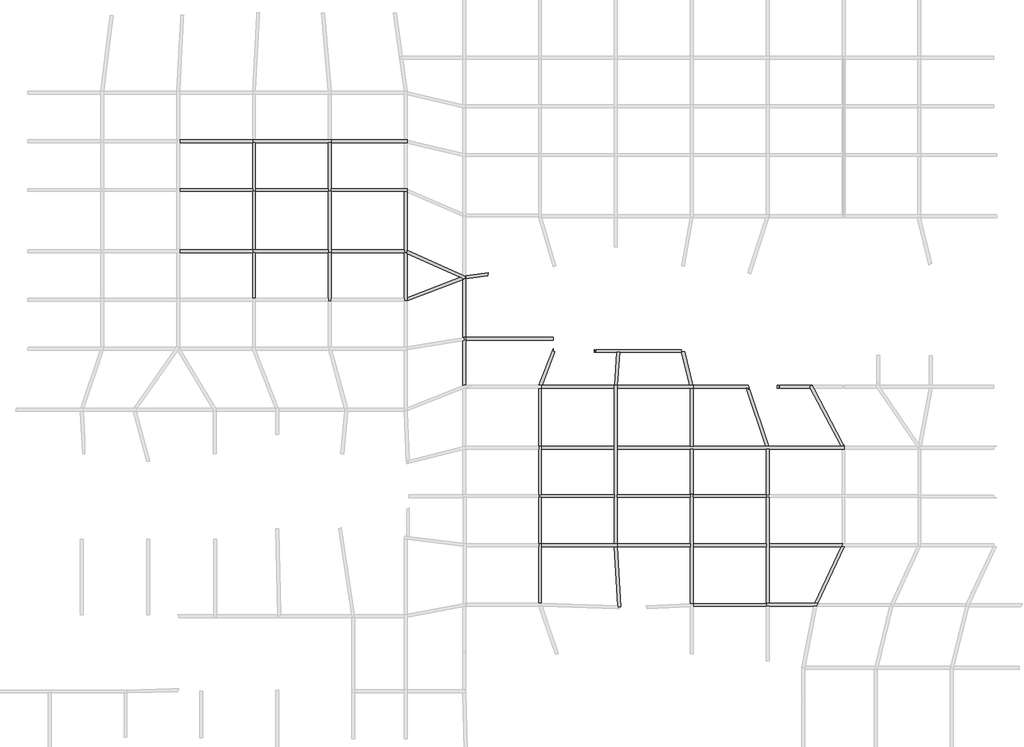
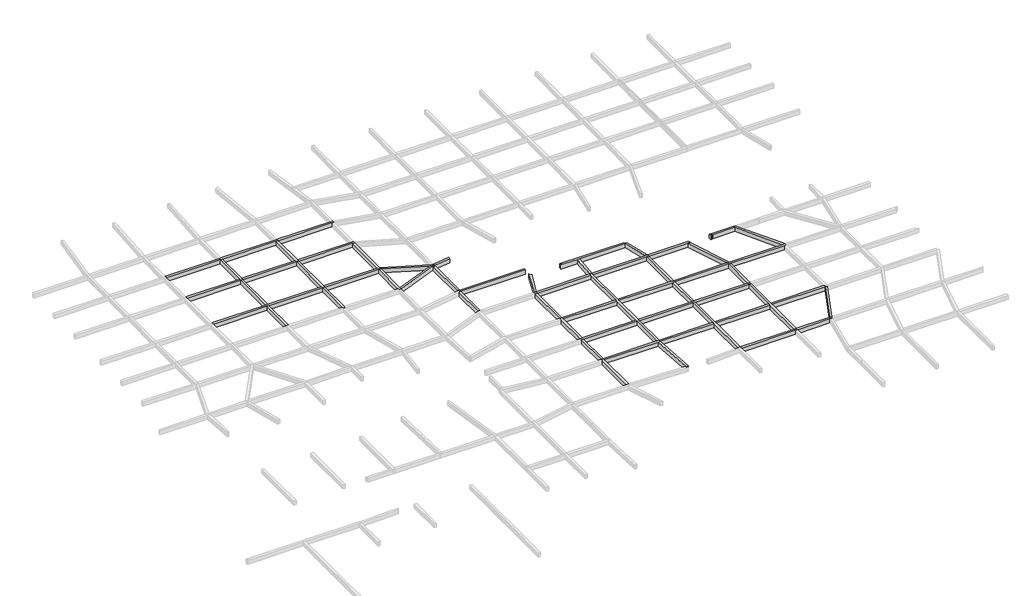
# One storey, part 7 of 15: 54 beams.
"""IFC4 building model written with IfcOpenShell, lengths in millimetres."""

from ifc_helpers import new_model, si_unit, frame, origin, place, context, project, spatial, polyline, outline, extrude, faceted_brep, element, save

model = new_model("IFC4")

# Units and contexts
model_context = context("Model", 3, world=origin())
ifc_project = project(units=[si_unit("LENGTHUNIT", "METRE", prefix="MILLI")], contexts=[model_context])

# Site, building, storey
site = spatial("IfcSite", under=ifc_project)
building = spatial("IfcBuilding", under=site)
storey = spatial("IfcBuildingStorey", under=building, Name="层高", Elevation=3300.0)

# Beams
placement = place(None, origin())
element("IfcBeam", 1, ObjectType="混凝土 - 矩形梁 : KL_beam", at=placement, inside=storey, context=model_context, shape_type="Brep", body=[
    faceted_brep([(161650.300938, 70392.1684205, 3300.0), (161350.300938, 70392.1684205, 3300.0), (161350.300938, 70092.1684205, 3300.0), (161350.300938, 64256.5260367, 3300.0), (161650.300938, 64256.5260367, 3300.0), (161650.300938, 70092.1684205, 3300.0), (161350.300938, 70392.1684205, 2700.0), (161350.300938, 70092.1684205, 2700.0), (161350.300938, 64256.5260367, 2700.0), (161650.300938, 70392.1684205, 2700.0), (161650.300938, 70092.1684205, 2700.0), (161650.300938, 64256.5260367, 2700.0)], [[[0, 1, 2, 3, 4, 5]], [[1, 6, 7, 8, 3, 2]], [[6, 9, 10, 11, 8, 7]], [[9, 0, 5, 4, 11, 10]], [[4, 3, 8, 11]], [[1, 0, 9, 6]]]),
])
element("IfcBeam", 2, ObjectType="混凝土 - 矩形梁 : KL_beam", at=placement, inside=storey, context=model_context, shape_type="Brep", body=[
    faceted_brep([(169458.3679569, 70092.1684205, 3300.0), (169450.3009381, 70246.0963088, 3300.0), (169442.6456231, 70392.1684205, 3300.0), (169150.3009381, 70392.1684205, 3300.0), (161650.300938, 70392.1684205, 3300.0), (161650.300938, 70092.1684205, 3300.0), (169157.9562531, 70092.1684205, 3300.0), (169458.3679569, 70092.1684205, 2700.0), (161650.300938, 70092.1684205, 2700.0), (169157.9562531, 70092.1684205, 2700.0), (169442.6456231, 70392.1684205, 2700.0), (169450.3009381, 70246.0963088, 2700.0), (161650.300938, 70392.1684205, 2700.0), (169150.3009381, 70392.1684205, 2700.0)], [[[0, 1, 2, 3, 4, 5, 6]], [[7, 0, 6, 5, 8, 9]], [[10, 11, 7, 9, 8, 12, 13]], [[2, 10, 13, 12, 4, 3]], [[5, 4, 12, 8]], [[2, 1, 0, 7, 11, 10]]]),
])
element("IfcBeam", 3, ObjectType="混凝土 - 矩形梁 : KL_beam", at=placement, inside=storey, context=model_context, shape_type="Brep", body=[
    faceted_brep([(169458.3679569, 70092.1684205, 3300.0), (169157.9562531, 70092.1684205, 3300.0), (169477.2686164, 63999.3255706, 3300.0), (169481.9445066, 63910.1042703, 3300.0), (169782.3562104, 63910.1042703, 3300.0), (169157.9562531, 70092.1684205, 2700.0), (169477.2686164, 63999.3255706, 2700.0), (169481.9445066, 63910.1042703, 2700.0), (169458.3679569, 70092.1684205, 2700.0), (169782.3562104, 63910.1042703, 2700.0)], [[[0, 1, 2, 3, 4]], [[1, 5, 6, 7, 3, 2]], [[5, 8, 9, 7, 6]], [[8, 0, 4, 9]], [[1, 0, 8, 5]], [[4, 3, 7, 9]]]),
])
element("IfcBeam", 4, ObjectType="混凝土 - 矩形梁 : KL_beam", at=placement, inside=storey, context=model_context, shape_type="Brep", body=[
    faceted_brep([(184765.5848537, 64245.2581831, 3300.0), (184765.5848537, 64242.1684205, 3300.0), (184765.5848537, 63945.2581831, 3300.0), (185065.5848537, 63945.2581831, 3300.0), (189579.4798373, 63945.2581831, 3300.0), (189910.8814312, 63945.2581831, 3300.0), (190050.2396546, 64242.1684205, 3300.0), (190051.6898701, 64245.2581831, 3300.0), (189720.2882761, 64245.2581831, 3300.0), (185065.5848537, 64245.2581831, 3300.0), (184765.5848537, 64245.2581831, 2700.0), (190051.6898701, 64245.2581831, 2700.0), (189720.2882761, 64245.2581831, 2700.0), (185065.5848537, 64245.2581831, 2700.0), (184765.5848537, 63945.2581831, 2700.0), (184765.5848537, 64242.1684205, 2700.0), (190050.2396546, 64242.1684205, 2700.0), (189910.8814312, 63945.2581831, 2700.0), (189579.4798373, 63945.2581831, 2700.0), (185065.5848537, 63945.2581831, 2700.0)], [[[0, 1, 2, 3, 4, 5, 6, 7, 8, 9]], [[10, 0, 9, 8, 7, 11, 12, 13]], [[14, 15, 10, 13, 12, 11, 16, 17, 18, 19]], [[2, 14, 19, 18, 17, 5, 4, 3]], [[2, 1, 0, 10, 15, 14]], [[7, 6, 5, 17, 16, 11]]]),
])
element("IfcBeam", 5, ObjectType="混凝土 - 矩形梁 : KL_beam", at=placement, inside=storey, context=model_context, shape_type="Brep", body=[
    faceted_brep([(184765.5848537, 64245.2581831, 3300.0), (185065.5848537, 64245.2581831, 3300.0), (185065.5848537, 70090.9378389, 3300.0), (185065.5848537, 70390.9378389, 3300.0), (185065.5848537, 75145.2581831, 3300.0), (184765.5848537, 75145.2581831, 3300.0), (184765.5848537, 70392.1684205, 3300.0), (184765.5848537, 70092.1684205, 3300.0), (185065.5848537, 64245.2581831, 2700.0), (185065.5848537, 70090.9378389, 2700.0), (185065.5848537, 70390.9378389, 2700.0), (185065.5848537, 75145.2581831, 2700.0), (184765.5848537, 64245.2581831, 2700.0), (184765.5848537, 70092.1684205, 2700.0), (184765.5848537, 70392.1684205, 2700.0), (184765.5848537, 75145.2581831, 2700.0)], [[[0, 1, 2, 3, 4, 5, 6, 7]], [[1, 8, 9, 10, 11, 4, 3, 2]], [[8, 12, 13, 14, 15, 11, 10, 9]], [[12, 0, 7, 6, 5, 15, 14, 13]], [[1, 0, 12, 8]], [[5, 4, 11, 15]]]),
])
element("IfcBeam", 6, ObjectType="混凝土 - 矩形梁 : KL_beam", at=placement, inside=storey, context=model_context, shape_type="Brep", body=[
    faceted_brep([(185065.5848537, 70390.9378389, 3300.0), (185065.5848537, 70090.9378389, 3300.0), (192464.0250307, 70090.9378389, 3300.0), (192604.8334695, 70390.9378389, 3300.0), (192550.1300471, 70390.9378389, 3300.0), (185065.5848537, 70090.9378389, 2700.0), (192464.0250307, 70090.9378389, 2700.0), (185065.5848537, 70390.9378389, 2700.0), (192550.1300471, 70390.9378389, 2700.0), (192604.8334695, 70390.9378389, 2700.0)], [[[0, 1, 2, 3, 4]], [[1, 5, 6, 2]], [[5, 7, 8, 9, 6]], [[7, 0, 4, 3, 9, 8]], [[1, 0, 7, 5]], [[3, 2, 6, 9]]]),
])
element("IfcBeam", 7, ObjectType="混凝土 - 矩形梁 : KL_beam", at=placement, inside=storey, context=model_context, shape_type="SweptSolid", body=[
    extrude(outline(polyline([(192464.0250307, 70090.9378389), (192795.4266246, 70090.9378389), (190051.6898701, 64245.2581831), (189720.2882761, 64245.2581831), (192464.0250307, 70090.9378389)])), frame((0.0, 0.0, 2700.0), z_axis=(0.0, 0.0, 1.0), x_axis=(1.0, 0.0, 0.0)), (0.0, 0.0, 1.0), 600.0),
])
element("IfcBeam", 8, ObjectType="混凝土 - 矩形梁 : KL_beam", at=placement, inside=storey, context=model_context, shape_type="Brep", body=[
    faceted_brep([(185065.5848537, 63942.1684205, 3300.0), (185065.5848537, 63945.2581831, 3300.0), (184765.5848537, 63945.2581831, 3300.0), (184765.5848537, 64242.1684205, 3300.0), (177250.3009381, 64242.1684205, 3300.0), (177250.3009381, 63942.1684205, 3300.0), (184765.5848537, 63942.1684205, 3300.0), (185065.5848537, 63942.1684205, 2700.0), (177250.3009381, 63942.1684205, 2700.0), (184765.5848537, 63942.1684205, 2700.0), (185065.5848537, 63945.2581831, 2700.0), (177250.3009381, 64242.1684205, 2700.0), (184765.5848537, 64242.1684205, 2700.0), (184765.5848537, 63945.2581831, 2700.0)], [[[0, 1, 2, 3, 4, 5, 6]], [[7, 0, 6, 5, 8, 9]], [[10, 7, 9, 8, 11, 12, 13]], [[3, 12, 11, 4]], [[0, 7, 10, 1]], [[13, 2, 1, 10]], [[2, 13, 12, 3]], [[5, 4, 11, 8]]]),
])
element("IfcBeam", 9, ObjectType="混凝土 - 矩形梁 : KL_beam", at=placement, inside=storey, context=model_context, shape_type="Brep", body=[
    faceted_brep([(176950.3009381, 75492.1684205, 3300.0), (176950.3009381, 75445.2581831, 3300.0), (176950.3009381, 75145.2581831, 3300.0), (176950.3009381, 70392.1684205, 3300.0), (176950.3009381, 70092.1684205, 3300.0), (176950.3009381, 64242.1684205, 3300.0), (177096.3665098, 64242.1684205, 3300.0), (177250.3009381, 64250.249233, 3300.0), (177250.3009381, 70092.1684205, 3300.0), (177250.3009381, 70392.1684205, 3300.0), (177250.3009381, 75145.2581831, 3300.0), (177250.3009381, 75445.2581831, 3300.0), (177250.3009381, 75492.1684205, 3300.0), (177250.3009381, 75492.1684205, 2700.0), (177250.3009381, 64250.249233, 2700.0), (177250.3009381, 70092.1684205, 2700.0), (177250.3009381, 70392.1684205, 2700.0), (177250.3009381, 75145.2581831, 2700.0), (177250.3009381, 75445.2581831, 2700.0), (176950.3009381, 64242.1684205, 2700.0), (176950.3009381, 70092.1684205, 2700.0), (176950.3009381, 70392.1684205, 2700.0), (176950.3009381, 75145.2581831, 2700.0), (176950.3009381, 75445.2581831, 2700.0), (176950.3009381, 75492.1684205, 2700.0), (177096.3665098, 64242.1684205, 2700.0)], [[[0, 1, 2, 3, 4, 5, 6, 7, 8, 9, 10, 11, 12]], [[13, 12, 11, 10, 9, 8, 7, 14, 15, 16, 17, 18]], [[19, 20, 21, 22, 23, 24, 13, 18, 17, 16, 15, 14, 25]], [[5, 4, 3, 2, 1, 0, 24, 23, 22, 21, 20, 19]], [[5, 19, 25, 6]], [[7, 6, 25, 14]], [[0, 12, 13, 24]]]),
])
element("IfcBeam", 10, ObjectType="混凝土 - 矩形梁 : KL_beam", at=placement, inside=storey, context=model_context, shape_type="SweptSolid", body=[
    extrude(outline(polyline([(184765.5848537, 70392.1684205), (184765.5848537, 70092.1684205), (177250.3009381, 70092.1684205), (177250.3009381, 70392.1684205), (184765.5848537, 70392.1684205)])), frame((0.0, 0.0, 2700.0), z_axis=(0.0, 0.0, 1.0), x_axis=(1.0, 0.0, 0.0)), (0.0, 0.0, 1.0), 600.0),
])
element("IfcBeam", 11, ObjectType="混凝土 - 矩形梁 : KL_beam", at=placement, inside=storey, context=model_context, shape_type="Brep", body=[
    faceted_brep([(192790.538789, 80092.1684205, 3300.0), (192790.538789, 80392.1684205, 3300.0), (192451.2603083, 80392.1684205, 3300.0), (185023.3152634, 80392.1684205, 3300.0), (184706.730176, 80392.1684205, 3300.0), (177250.3009381, 80392.1684205, 3300.0), (176950.3009381, 80392.1684205, 3300.0), (169450.3009381, 80392.1684205, 3300.0), (169450.3009381, 80092.1684205, 3300.0), (176950.3009381, 80092.1684205, 3300.0), (177250.3009381, 80092.1684205, 3300.0), (184765.5848537, 80092.1684205, 3300.0), (185065.5848537, 80092.1684205, 3300.0), (192550.1300471, 80092.1684205, 3300.0), (192790.538789, 80392.1684205, 2700.0), (192451.2603083, 80392.1684205, 2700.0), (185023.3152634, 80392.1684205, 2700.0), (184706.730176, 80392.1684205, 2700.0), (177250.3009381, 80392.1684205, 2700.0), (176950.3009381, 80392.1684205, 2700.0), (169450.3009381, 80392.1684205, 2700.0), (192790.538789, 80092.1684205, 2700.0), (192550.1300471, 80092.1684205, 2700.0), (185065.5848537, 80092.1684205, 2700.0), (184765.5848537, 80092.1684205, 2700.0), (177250.3009381, 80092.1684205, 2700.0), (176950.3009381, 80092.1684205, 2700.0), (169450.3009381, 80092.1684205, 2700.0)], [[[0, 1, 2, 3, 4, 5, 6, 7, 8, 9, 10, 11, 12, 13]], [[1, 14, 15, 16, 17, 18, 19, 20, 7, 6, 5, 4, 3, 2]], [[14, 21, 22, 23, 24, 25, 26, 27, 20, 19, 18, 17, 16, 15]], [[21, 0, 13, 12, 11, 10, 9, 8, 27, 26, 25, 24, 23, 22]], [[8, 7, 20, 27]], [[0, 21, 14, 1]]]),
])
element("IfcBeam", 12, ObjectType="混凝土 - 矩形梁 : KL_beam", at=placement, inside=storey, context=model_context, shape_type="SweptSolid", body=[
    extrude(outline(polyline([(177250.3009381, 75492.1684205), (176950.3009381, 75492.1684205), (176950.3009381, 80092.1684205), (177250.3009381, 80092.1684205), (177250.3009381, 75492.1684205)])), frame((0.0, 0.0, 2700.0), z_axis=(0.0, 0.0, 1.0), x_axis=(1.0, 0.0, 0.0)), (0.0, 0.0, 1.0), 600.0),
])
element("IfcBeam", 13, ObjectType="混凝土 - 矩形梁 : KL_beam", at=placement, inside=storey, context=model_context, shape_type="SweptSolid", body=[
    extrude(outline(polyline([(184765.5848537, 80092.1684205), (185065.5848537, 80092.1684205), (185065.5848537, 75445.2581831), (184765.5848537, 75445.2581831), (184765.5848537, 80092.1684205)])), frame((0.0, 0.0, 2700.0), z_axis=(0.0, 0.0, 1.0), x_axis=(1.0, 0.0, 0.0)), (0.0, 0.0, 1.0), 600.0),
])
element("IfcBeam", 14, ObjectType="混凝土 - 矩形梁 : KL_beam", at=placement, inside=storey, context=model_context, shape_type="Brep", body=[
    faceted_brep([(169150.3009381, 70392.1684205, 3300.0), (169442.6456231, 70392.1684205, 3300.0), (169450.3009381, 70246.0963088, 3300.0), (169450.3009381, 70392.1684205, 3300.0), (169450.3009381, 75145.2581831, 3300.0), (169450.3009381, 75445.2581831, 3300.0), (169450.3009381, 80092.1684205, 3300.0), (169450.3009381, 80392.1684205, 3300.0), (169450.3009381, 86368.5594398, 3300.0), (169450.3009381, 86668.5594398, 3300.0), (169160.4236752, 86668.5594398, 3300.0), (169150.3009381, 86668.5594398, 3300.0), (169150.3009381, 86368.5594398, 3300.0), (169150.3009381, 80384.9176514, 3300.0), (169150.3009381, 80084.9176514, 3300.0), (169150.3009381, 75445.2581831, 3300.0), (169150.3009381, 75145.2581831, 3300.0), (169150.3009381, 70392.1684205, 2700.0), (169150.3009381, 86668.5594398, 2700.0), (169150.3009381, 86368.5594398, 2700.0), (169150.3009381, 80384.9176514, 2700.0), (169150.3009381, 80084.9176514, 2700.0), (169150.3009381, 75445.2581831, 2700.0), (169150.3009381, 75145.2581831, 2700.0), (169442.6456231, 70392.1684205, 2700.0), (169160.4236752, 86668.5594398, 2700.0), (169450.3009381, 86668.5594398, 2700.0), (169450.3009381, 86368.5594398, 2700.0), (169450.3009381, 80392.1684205, 2700.0), (169450.3009381, 80092.1684205, 2700.0), (169450.3009381, 75445.2581831, 2700.0), (169450.3009381, 75145.2581831, 2700.0), (169450.3009381, 70392.1684205, 2700.0), (169450.3009381, 70246.0963088, 2700.0)], [[[0, 1, 2, 3, 4, 5, 6, 7, 8, 9, 10, 11, 12, 13, 14, 15, 16]], [[17, 0, 16, 15, 14, 13, 12, 11, 18, 19, 20, 21, 22, 23]], [[24, 17, 23, 22, 21, 20, 19, 18, 25, 26, 27, 28, 29, 30, 31, 32, 33]], [[2, 33, 32, 31, 30, 29, 28, 27, 26, 9, 8, 7, 6, 5, 4, 3]], [[24, 1, 0, 17]], [[1, 24, 33, 2]], [[11, 10, 9, 26, 25, 18]]]),
])
element("IfcBeam", 15, ObjectType="混凝土 - 矩形梁 : KL_beam", at=placement, inside=storey, context=model_context, shape_type="Brep", body=[
    faceted_brep([(184765.5848537, 75145.2581831, 3300.0), (184765.5848537, 75445.2581831, 3300.0), (177250.3009381, 75445.2581831, 3300.0), (177250.3009381, 75145.2581831, 3300.0), (184765.5848537, 75445.2581831, 2700.0), (177250.3009381, 75445.2581831, 2700.0), (184765.5848537, 75145.2581831, 2700.0), (177250.3009381, 75145.2581831, 2700.0)], [[[0, 1, 2, 3]], [[1, 4, 5, 2]], [[4, 6, 7, 5]], [[6, 0, 3, 7]], [[1, 0, 6, 4]], [[3, 2, 5, 7]]]),
    faceted_brep([(176950.3009381, 75445.2581831, 3300.0), (176950.3009381, 75145.2581831, 3300.0), (176950.3009381, 75145.2581831, 2700.0), (176950.3009381, 75445.2581831, 2700.0), (169450.3009381, 75145.2581831, 3300.0), (169450.3009381, 75445.2581831, 3300.0), (169450.3009381, 75445.2581831, 2700.0), (169450.3009381, 75145.2581831, 2700.0)], [[[0, 1, 2, 3]], [[4, 5, 6, 7]], [[1, 0, 5, 4]], [[0, 3, 6, 5]], [[3, 2, 7, 6]], [[2, 1, 4, 7]]]),
    faceted_brep([(161350.300938, 75445.2581831, 3300.0), (161350.300938, 75145.2581831, 3300.0), (161650.300938, 75145.2581831, 3300.0), (169150.3009381, 75145.2581831, 3300.0), (169150.3009381, 75445.2581831, 3300.0), (161650.300938, 75445.2581831, 3300.0), (161350.300938, 75445.2581831, 2700.0), (169150.3009381, 75445.2581831, 2700.0), (161650.300938, 75445.2581831, 2700.0), (161350.300938, 75145.2581831, 2700.0), (169150.3009381, 75145.2581831, 2700.0), (161650.300938, 75145.2581831, 2700.0)], [[[0, 1, 2, 3, 4, 5]], [[6, 0, 5, 4, 7, 8]], [[9, 6, 8, 7, 10, 11]], [[1, 9, 11, 10, 3, 2]], [[4, 3, 10, 7]], [[1, 0, 6, 9]]]),
])
element("IfcBeam", 16, ObjectType="混凝土 - 矩形梁 : KL_beam", at=placement, inside=storey, context=model_context, shape_type="Brep", body=[
    faceted_brep([(161650.300938, 80384.9176514, 3300.0), (161350.300938, 80384.9176514, 3300.0), (161350.300938, 80084.9176514, 3300.0), (161350.300938, 75445.2581831, 3300.0), (161650.300938, 75445.2581831, 3300.0), (161650.300938, 80084.9176514, 3300.0), (161650.300938, 80384.9176514, 2700.0), (161650.300938, 75445.2581831, 2700.0), (161650.300938, 80084.9176514, 2700.0), (161350.300938, 80384.9176514, 2700.0), (161350.300938, 75445.2581831, 2700.0), (161350.300938, 80084.9176514, 2700.0)], [[[0, 1, 2, 3, 4, 5]], [[6, 0, 5, 4, 7, 8]], [[9, 6, 8, 7, 10, 11]], [[1, 9, 11, 10, 3, 2]], [[4, 3, 10, 7]], [[1, 0, 6, 9]]]),
])
element("IfcBeam", 17, ObjectType="混凝土 - 矩形梁 : KL_beam", at=placement, inside=storey, context=model_context, shape_type="SweptSolid", body=[
    extrude(outline(polyline([(161650.300938, 70392.1684205), (161350.300938, 70392.1684205), (161350.300938, 75145.2581831), (161650.300938, 75145.2581831), (161650.300938, 70392.1684205)])), frame((0.0, 0.0, 2700.0), z_axis=(0.0, 0.0, 1.0), x_axis=(1.0, 0.0, 0.0)), (0.0, 0.0, 1.0), 600.0),
])
element("IfcBeam", 18, ObjectType="混凝土 - 矩形梁 : KL_beam", at=placement, inside=storey, context=model_context, shape_type="SweptSolid", body=[
    extrude(outline(polyline([(169458.3679569, 70092.1684205), (169450.3009381, 70246.0963088), (169450.3009381, 70392.1684205), (176950.3009381, 70392.1684205), (176950.3009381, 70092.1684205), (169458.3679569, 70092.1684205)])), frame((0.0, 0.0, 2700.0), z_axis=(0.0, 0.0, 1.0), x_axis=(1.0, 0.0, 0.0)), (0.0, 0.0, 1.0), 600.0),
])
element("IfcBeam", 19, ObjectType="混凝土 - 矩形梁 : KL_beam", at=placement, inside=storey, context=model_context, shape_type="Brep", body=[
    faceted_brep([(131950.3009381, 111892.3894162, 3300.0), (131950.3009381, 111592.3894162, 3300.0), (132250.3009381, 111592.3894162, 3300.0), (139750.3009381, 111592.3894162, 3300.0), (140050.3009381, 111592.3894162, 3300.0), (140050.3009381, 111892.3894162, 3300.0), (139750.3009381, 111892.3894162, 3300.0), (132250.3009381, 111892.3894162, 3300.0), (131950.3009381, 111892.3894162, 2700.0), (140050.3009381, 111892.3894162, 2700.0), (139750.3009381, 111892.3894162, 2700.0), (132250.3009381, 111892.3894162, 2700.0), (131950.3009381, 111592.3894162, 2700.0), (140050.3009381, 111592.3894162, 2700.0), (139750.3009381, 111592.3894162, 2700.0), (132250.3009381, 111592.3894162, 2700.0)], [[[0, 1, 2, 3, 4, 5, 6, 7]], [[8, 0, 7, 6, 5, 9, 10, 11]], [[12, 8, 11, 10, 9, 13, 14, 15]], [[1, 12, 15, 14, 13, 4, 3, 2]], [[1, 0, 8, 12]], [[5, 4, 13, 9]]]),
])
element("IfcBeam", 20, ObjectType="混凝土 - 矩形梁 : KL_beam", at=placement, inside=storey, context=model_context, shape_type="Brep", body=[
    faceted_brep([(131950.3009381, 106592.3894162, 3300.0), (132250.3009381, 106592.3894162, 3300.0), (132250.3009381, 106892.3894162, 3300.0), (132250.3009381, 111592.3894162, 3300.0), (131950.3009381, 111592.3894162, 3300.0), (131950.3009381, 106892.3894162, 3300.0), (132250.3009381, 106592.3894162, 2700.0), (132250.3009381, 106892.3894162, 2700.0), (132250.3009381, 111592.3894162, 2700.0), (131950.3009381, 106592.3894162, 2700.0), (131950.3009381, 106892.3894162, 2700.0), (131950.3009381, 111592.3894162, 2700.0)], [[[0, 1, 2, 3, 4, 5]], [[1, 6, 7, 8, 3, 2]], [[6, 9, 10, 11, 8, 7]], [[9, 0, 5, 4, 11, 10]], [[4, 3, 8, 11]], [[1, 0, 9, 6]]]),
])
element("IfcBeam", 21, ObjectType="混凝土 - 矩形梁 : KL_beam", at=placement, inside=storey, context=model_context, shape_type="Brep", body=[
    faceted_brep([(139750.3009381, 106592.3894162, 3300.0), (140050.3009381, 106592.3894162, 3300.0), (140050.3009381, 106892.3894162, 3300.0), (140050.3009381, 111592.3894162, 3300.0), (139750.3009381, 111592.3894162, 3300.0), (139750.3009381, 106892.3894162, 3300.0), (140050.3009381, 106592.3894162, 2700.0), (140050.3009381, 106892.3894162, 2700.0), (140050.3009381, 111592.3894162, 2700.0), (139750.3009381, 106592.3894162, 2700.0), (139750.3009381, 106892.3894162, 2700.0), (139750.3009381, 111592.3894162, 2700.0)], [[[0, 1, 2, 3, 4, 5]], [[1, 6, 7, 8, 3, 2]], [[6, 9, 10, 11, 8, 7]], [[9, 0, 5, 4, 11, 10]], [[4, 3, 8, 11]], [[1, 0, 9, 6]]]),
])
element("IfcBeam", 22, ObjectType="混凝土 - 矩形梁 : KL_beam", at=placement, inside=storey, context=model_context, shape_type="SweptSolid", body=[
    extrude(outline(polyline([(132250.3009381, 106592.3894162), (132250.3009381, 106892.3894162), (139750.3009381, 106892.3894162), (139750.3009381, 106592.3894162), (132250.3009381, 106592.3894162)])), frame((0.0, 0.0, 2700.0), z_axis=(0.0, 0.0, 1.0), x_axis=(1.0, 0.0, 0.0)), (0.0, 0.0, 1.0), 600.0),
])
element("IfcBeam", 23, ObjectType="混凝土 - 矩形梁 : KL_beam", at=placement, inside=storey, context=model_context, shape_type="Brep", body=[
    faceted_brep([(147850.2032763, 111592.3894162, 3300.0), (147850.2032763, 111861.4143495, 3300.0), (147850.2032763, 111892.3894162, 3300.0), (147550.2032763, 111892.3894162, 3300.0), (140050.3009381, 111892.3894162, 3300.0), (140050.3009381, 111592.3894162, 3300.0), (147550.2032763, 111592.3894162, 3300.0), (147850.2032763, 111892.3894162, 2700.0), (147550.2032763, 111892.3894162, 2700.0), (140050.3009381, 111892.3894162, 2700.0), (147850.2032763, 111861.4143495, 2700.0), (147850.2032763, 111592.3894162, 2700.0), (147550.2032763, 111592.3894162, 2700.0), (140050.3009381, 111592.3894162, 2700.0)], [[[0, 1, 2, 3, 4, 5, 6]], [[2, 7, 8, 9, 4, 3]], [[7, 10, 11, 12, 13, 9, 8]], [[11, 0, 6, 5, 13, 12]], [[5, 4, 9, 13]], [[2, 1, 0, 11, 10, 7]]]),
])
element("IfcBeam", 24, ObjectType="混凝土 - 矩形梁 : KL_beam", at=placement, inside=storey, context=model_context, shape_type="Brep", body=[
    faceted_brep([(147850.2032763, 106592.3894162, 3300.0), (147850.2032763, 106840.5198943, 3300.0), (147850.2032763, 106892.3894162, 3300.0), (147550.2032763, 106892.3894162, 3300.0), (140050.3009381, 106892.3894162, 3300.0), (140050.3009381, 106592.3894162, 3300.0), (147550.2032763, 106592.3894162, 3300.0), (147668.8470787, 106592.3894162, 3300.0), (147850.2032763, 106592.3894162, 2700.0), (140050.3009381, 106592.3894162, 2700.0), (147550.2032763, 106592.3894162, 2700.0), (147668.8470787, 106592.3894162, 2700.0), (147850.2032763, 106892.3894162, 2700.0), (147850.2032763, 106840.5198943, 2700.0), (140050.3009381, 106892.3894162, 2700.0), (147550.2032763, 106892.3894162, 2700.0)], [[[0, 1, 2, 3, 4, 5, 6, 7]], [[8, 0, 7, 6, 5, 9, 10, 11]], [[12, 13, 8, 11, 10, 9, 14, 15]], [[2, 12, 15, 14, 4, 3]], [[5, 4, 14, 9]], [[2, 1, 0, 8, 13, 12]]]),
])
element("IfcBeam", 25, ObjectType="混凝土 - 矩形梁 : KL_beam", at=placement, inside=storey, context=model_context, shape_type="Brep", body=[
    faceted_brep([(147550.2032763, 100292.3894162, 3300.0), (147668.0058777, 100292.3894162, 3300.0), (147850.2032763, 100292.3894162, 3300.0), (147850.2032763, 100539.3742818, 3300.0), (147850.2032763, 106513.1028536, 3300.0), (147668.8470787, 106592.3894162, 3300.0), (147550.2032763, 106592.3894162, 3300.0), (147550.2032763, 100592.3894162, 3300.0), (147550.2032763, 106592.3894162, 2700.0), (147550.2032763, 100592.3894162, 2700.0), (147550.2032763, 100292.3894162, 2700.0), (147850.2032763, 100292.3894162, 2700.0), (147668.0058777, 100292.3894162, 2700.0), (147668.8470787, 106592.3894162, 2700.0), (147850.2032763, 106513.1028536, 2700.0), (147850.2032763, 100539.3742818, 2700.0)], [[[0, 1, 2, 3, 4, 5, 6, 7]], [[6, 8, 9, 10, 0, 7]], [[11, 12, 10, 9, 8, 13, 14, 15]], [[2, 11, 15, 14, 4, 3]], [[8, 6, 5, 13]], [[5, 4, 14, 13]], [[2, 1, 0, 10, 12, 11]]]),
])
element("IfcBeam", 26, ObjectType="混凝土 - 矩形梁 : KL_beam", at=placement, inside=storey, context=model_context, shape_type="Brep", body=[
    faceted_brep([(139750.3009381, 100292.3894162, 3300.0), (140050.3009381, 100292.3894162, 3300.0), (140050.3009381, 100592.3894162, 3300.0), (140050.3009381, 106592.3894162, 3300.0), (139750.3009381, 106592.3894162, 3300.0), (139750.3009381, 100592.3894162, 3300.0), (140050.3009381, 100292.3894162, 2700.0), (140050.3009381, 100592.3894162, 2700.0), (140050.3009381, 106592.3894162, 2700.0), (139750.3009381, 100292.3894162, 2700.0), (139750.3009381, 100592.3894162, 2700.0), (139750.3009381, 106592.3894162, 2700.0)], [[[0, 1, 2, 3, 4, 5]], [[1, 6, 7, 8, 3, 2]], [[6, 9, 10, 11, 8, 7]], [[9, 0, 5, 4, 11, 10]], [[4, 3, 8, 11]], [[1, 0, 9, 6]]]),
])
element("IfcBeam", 27, ObjectType="混凝土 - 矩形梁 : KL_beam", at=placement, inside=storey, context=model_context, shape_type="SweptSolid", body=[
    extrude(outline(polyline([(147550.2032763, 100592.3894162), (147550.2032763, 100292.3894162), (140050.3009381, 100292.3894162), (140050.3009381, 100592.3894162), (147550.2032763, 100592.3894162)])), frame((0.0, 0.0, 2700.0), z_axis=(0.0, 0.0, 1.0), x_axis=(1.0, 0.0, 0.0)), (0.0, 0.0, 1.0), 600.0),
])
element("IfcBeam", 28, ObjectType="混凝土 - 矩形梁 : KL_beam", at=placement, inside=storey, context=model_context, shape_type="Brep", body=[
    faceted_brep([(147850.2032763, 100539.3742818, 3300.0), (147850.2032763, 100292.3894162, 3300.0), (147668.0058777, 100292.3894162, 3300.0), (147850.2032763, 100210.3944563, 3300.0), (153310.1557551, 97753.2321258, 3300.0), (153695.684915, 97579.7310317, 3300.0), (153727.18388, 97565.5554376, 3300.0), (153741.0642282, 97596.3983497, 3300.0), (153741.4601305, 97597.2780667, 3300.0), (153850.3009381, 97839.1284443, 3300.0), (153550.3009381, 97974.1385386, 3300.0), (147668.0058777, 100292.3894162, 2700.0), (147850.2032763, 100210.3944563, 2700.0), (153310.1557551, 97753.2321258, 2700.0), (153695.684915, 97579.7310317, 2700.0), (153727.18388, 97565.5554376, 2700.0), (147850.2032763, 100292.3894162, 2700.0), (147850.2032763, 100539.3742818, 2700.0), (153550.3009381, 97974.1385386, 2700.0), (153850.3009381, 97839.1284443, 2700.0), (153741.4601305, 97597.2780667, 2700.0), (153741.0642282, 97596.3983497, 2700.0)], [[[0, 1, 2, 3, 4, 5, 6, 7, 8, 9, 10]], [[2, 11, 12, 13, 14, 15, 6, 5, 4, 3]], [[16, 17, 18, 19, 20, 21, 15, 14, 13, 12, 11]], [[17, 0, 10, 9, 19, 18]], [[16, 1, 0, 17]], [[1, 16, 11, 2]], [[9, 8, 7, 6, 15, 21, 20, 19]]]),
])
element("IfcBeam", 29, ObjectType="混凝土 - 矩形梁 : KL_beam", at=placement, inside=storey, context=model_context, shape_type="Brep", body=[
    faceted_brep([(147550.2032763, 95338.9797898, 3300.0), (147850.2032763, 95338.9797898, 3300.0), (147850.2032763, 95660.2659592, 3300.0), (147850.2032763, 100210.3944563, 3300.0), (147668.0058777, 100292.3894162, 3300.0), (147550.2032763, 100292.3894162, 3300.0), (147550.2032763, 95592.1233035, 3300.0), (147550.2032763, 100292.3894162, 2700.0), (147550.2032763, 95592.1233035, 2700.0), (147550.2032763, 95338.9797898, 2700.0), (147850.2032763, 95338.9797898, 2700.0), (147668.0058777, 100292.3894162, 2700.0), (147850.2032763, 100210.3944563, 2700.0), (147850.2032763, 95660.2659592, 2700.0)], [[[0, 1, 2, 3, 4, 5, 6]], [[5, 7, 8, 9, 0, 6]], [[10, 9, 8, 7, 11, 12, 13]], [[1, 10, 13, 12, 3, 2]], [[7, 5, 4, 11]], [[4, 3, 12, 11]], [[1, 0, 9, 10]]]),
])
element("IfcBeam", 30, ObjectType="混凝土 - 矩形梁 : KL_beam", at=placement, inside=storey, context=model_context, shape_type="Brep", body=[
    faceted_brep([(139750.3009381, 95292.1233035, 3300.0), (140050.3009381, 95292.1233035, 3300.0), (140050.3009381, 95592.1233035, 3300.0), (140050.3009381, 100292.3894162, 3300.0), (139750.3009381, 100292.3894162, 3300.0), (139750.3009381, 95592.1233035, 3300.0), (139750.3009381, 95292.1233035, 2700.0), (139750.3009381, 100292.3894162, 2700.0), (139750.3009381, 95592.1233035, 2700.0), (140050.3009381, 95292.1233035, 2700.0), (140050.3009381, 100292.3894162, 2700.0), (140050.3009381, 95592.1233035, 2700.0)], [[[0, 1, 2, 3, 4, 5]], [[6, 0, 5, 4, 7, 8]], [[9, 6, 8, 7, 10, 11]], [[1, 9, 11, 10, 3, 2]], [[4, 3, 10, 7]], [[1, 0, 6, 9]]]),
])
element("IfcBeam", 31, ObjectType="混凝土 - 矩形梁 : KL_beam", at=placement, inside=storey, context=model_context, shape_type="Brep", body=[
    faceted_brep([(131950.3009381, 100592.3894162, 3300.0), (131950.3009381, 100292.3894162, 3300.0), (132250.3009381, 100292.3894162, 3300.0), (139750.3009381, 100292.3894162, 3300.0), (139750.3009381, 100592.3894162, 3300.0), (132250.3009381, 100592.3894162, 3300.0), (131950.3009381, 100292.3894162, 2700.0), (132250.3009381, 100292.3894162, 2700.0), (139750.3009381, 100292.3894162, 2700.0), (131950.3009381, 100592.3894162, 2700.0), (132250.3009381, 100592.3894162, 2700.0), (139750.3009381, 100592.3894162, 2700.0)], [[[0, 1, 2, 3, 4, 5]], [[1, 6, 7, 8, 3, 2]], [[6, 9, 10, 11, 8, 7]], [[9, 0, 5, 4, 11, 10]], [[4, 3, 8, 11]], [[1, 0, 9, 6]]]),
])
element("IfcBeam", 32, ObjectType="混凝土 - 矩形梁 : KL_beam", at=placement, inside=storey, context=model_context, shape_type="SweptSolid", body=[
    extrude(outline(polyline([(131950.3009381, 100292.3894162), (132250.3009381, 100292.3894162), (132250.3009381, 95592.1233035), (131950.3009381, 95592.1233035), (131950.3009381, 100292.3894162)])), frame((0.0, 0.0, 2700.0), z_axis=(0.0, 0.0, 1.0), x_axis=(1.0, 0.0, 0.0)), (0.0, 0.0, 1.0), 600.0),
])
element("IfcBeam", 33, ObjectType="混凝土 - 矩形梁 : KL_beam", at=placement, inside=storey, context=model_context, shape_type="SweptSolid", body=[
    extrude(outline(polyline([(131950.3009381, 106592.3894162), (132250.3009381, 106592.3894162), (132250.3009381, 100592.3894162), (131950.3009381, 100592.3894162), (131950.3009381, 106592.3894162)])), frame((0.0, 0.0, 2700.0), z_axis=(0.0, 0.0, 1.0), x_axis=(1.0, 0.0, 0.0)), (0.0, 0.0, 1.0), 600.0),
])
element("IfcBeam", 34, ObjectType="混凝土 - 矩形梁 : KL_beam", at=placement, inside=storey, context=model_context, shape_type="SweptSolid", body=[
    extrude(outline(polyline([(124450.3009381, 100292.3894162), (124450.3009381, 100592.3894162), (131950.3009381, 100592.3894162), (131950.3009381, 100292.3894162), (124450.3009381, 100292.3894162)])), frame((0.0, 0.0, 2700.0), z_axis=(0.0, 0.0, 1.0), x_axis=(1.0, 0.0, 0.0)), (0.0, 0.0, 1.0), 600.0),
])
element("IfcBeam", 35, ObjectType="混凝土 - 矩形梁 : KL_beam", at=placement, inside=storey, context=model_context, shape_type="SweptSolid", body=[
    extrude(outline(polyline([(124450.3009381, 106592.3894162), (124450.3009381, 106892.3894162), (131950.3009381, 106892.3894162), (131950.3009381, 106592.3894162), (124450.3009381, 106592.3894162)])), frame((0.0, 0.0, 2700.0), z_axis=(0.0, 0.0, 1.0), x_axis=(1.0, 0.0, 0.0)), (0.0, 0.0, 1.0), 600.0),
])
element("IfcBeam", 36, ObjectType="混凝土 - 矩形梁 : KL_beam", at=placement, inside=storey, context=model_context, shape_type="Brep", body=[
    faceted_brep([(189203.3917758, 86541.0667552, 3300.0), (189287.8431053, 86381.1826239, 3300.0), (192451.2603083, 80392.1684205, 3300.0), (192790.538789, 80392.1684205, 3300.0), (192711.3752265, 80542.0416967, 3300.0), (192640.3009401, 80542.0416967, 3300.0), (192640.3009401, 80676.6002718, 3300.0), (189627.121586, 86381.1826239, 3300.0), (189468.6605892, 86681.1826239, 3300.0), (189203.3917758, 86541.0667552, 2700.0), (189287.8431053, 86381.1826239, 2700.0), (192451.2603083, 80392.1684205, 2700.0), (189468.6605892, 86681.1826239, 2700.0), (189627.121586, 86381.1826239, 2700.0), (192640.3009401, 80676.6002718, 2700.0), (192640.3009401, 80542.0416967, 2700.0), (192711.3752265, 80542.0416967, 2700.0), (192790.538789, 80392.1684205, 2700.0)], [[[0, 1, 2, 3, 4, 5, 6, 7, 8]], [[2, 1, 0, 9, 10, 11]], [[11, 10, 9, 12, 13, 14, 15, 16, 17]], [[3, 17, 16, 4]], [[3, 2, 11, 17]], [[8, 12, 9, 0]], [[5, 15, 14, 6]], [[15, 5, 4, 16]], [[12, 8, 7, 6, 14, 13]]]),
])
element("IfcBeam", 37, ObjectType="混凝土 - 矩形梁 : KL_beam", at=placement, inside=storey, context=model_context, shape_type="Brep", body=[
    faceted_brep([(153850.3009381, 97639.000065, 2700.0), (153850.3009381, 97639.000065, 3300.0), (153741.4601305, 97597.2780667, 3300.0), (153741.4601305, 97597.2780667, 2700.0), (153850.3009381, 97839.1284443, 2700.0), (153850.3009381, 97839.1284443, 3300.0)], [[[0, 1, 2, 3]], [[1, 0, 4, 5]], [[1, 5, 2]], [[4, 0, 3]], [[2, 5, 4, 3]]]),
    faceted_brep([(153695.684915, 97579.7310317, 3300.0), (153695.684915, 97579.7310317, 2700.0), (153550.3009381, 97645.1587131, 2700.0), (153310.1557551, 97753.2321258, 2700.0), (153310.1557551, 97753.2321258, 3300.0), (153550.3009381, 97645.1587131, 3300.0), (147850.2032763, 95660.2659592, 2700.0), (147850.2032763, 95660.2659592, 3300.0), (147850.2032763, 95338.9797898, 2700.0), (147850.2032763, 95338.9797898, 3300.0), (153550.3009381, 97524.0009231, 3300.0), (153550.3009381, 97524.0009231, 2700.0)], [[[0, 1, 2, 3, 4, 5]], [[4, 3, 6, 7]], [[7, 6, 8, 9]], [[9, 10, 0, 5, 4, 7]], [[0, 10, 9, 8, 11, 1]], [[1, 11, 8, 6, 3, 2]]]),
])
element("IfcBeam", 38, ObjectType="混凝土 - 矩形梁 : KL_beam", at=placement, inside=storey, context=model_context, shape_type="Brep", body=[
    faceted_brep([(156166.4670288, 98240.2147555, 2700.0), (156166.4670288, 98240.2147555, 3300.0), (156179.085005, 98150.4331897, 3300.0), (156179.085005, 98150.4331897, 2700.0), (153850.3009381, 97914.6988398, 3300.0), (153850.3009381, 97839.1284443, 3300.0), (153850.3009381, 97639.000065, 3300.0), (153741.4601305, 97597.2780667, 3300.0), (153741.0642282, 97596.3983497, 3300.0), (153850.3009381, 97611.750568, 3300.0), (156127.8219291, 97931.8352692, 3300.0), (156127.8219291, 98150.4331897, 3300.0), (153741.0642282, 97596.3983497, 2700.0), (153850.3009381, 97611.750568, 2700.0), (156127.8219291, 97931.8352692, 2700.0), (153850.3009381, 97914.6988398, 2700.0), (156127.8219291, 98150.4331897, 2700.0), (153741.4601305, 97597.2780667, 2700.0), (153850.3009381, 97639.000065, 2700.0), (153850.3009381, 97839.1284443, 2700.0)], [[[0, 1, 2, 3]], [[1, 4, 5, 6, 7, 8, 9, 10, 11, 2]], [[8, 12, 13, 14, 10, 9]], [[15, 0, 3, 16, 14, 13, 12, 17, 18, 19]], [[1, 0, 15, 4]], [[12, 8, 7, 17]], [[4, 15, 19, 18, 6, 5]], [[6, 18, 17, 7]], [[16, 11, 10, 14]], [[11, 16, 3, 2]]]),
])
element("IfcBeam", 39, ObjectType="混凝土 - 矩形梁 : KL_beam", at=placement, inside=storey, context=model_context, shape_type="SweptSolid", body=[
    extrude(outline(polyline([(153695.684915, 97579.7310317), (153727.18388, 97565.5554376), (153741.0642282, 97596.3983497), (153850.3009381, 97611.750568), (153850.3009381, 91592.168885), (153687.8894584, 91592.168885), (153550.3009381, 91569.2428953), (153550.3009381, 97524.0009231), (153695.684915, 97579.7310317)])), frame((0.0, 0.0, 2700.0), z_axis=(0.0, 0.0, 1.0), x_axis=(1.0, 0.0, 0.0)), (0.0, 0.0, 1.0), 600.0),
])
element("IfcBeam", 40, ObjectType="混凝土 - 矩形梁 : KL_beam", at=placement, inside=storey, context=model_context, shape_type="SweptSolid", body=[
    extrude(outline(polyline([(124450.3009381, 111592.3894162), (124450.3009381, 111892.3894162), (131950.3009381, 111892.3894162), (131950.3009381, 111592.3894162), (124450.3009381, 111592.3894162)])), frame((0.0, 0.0, 2700.0), z_axis=(0.0, 0.0, 1.0), x_axis=(1.0, 0.0, 0.0)), (0.0, 0.0, 1.0), 600.0),
])
element("IfcBeam", 41, ObjectType="混凝土 - 矩形梁 : KL_beam", at=placement, inside=storey, context=model_context, shape_type="SweptSolid", body=[
    extrude(outline(polyline([(161350.300938, 86368.5594398), (161650.300938, 86368.5594398), (161650.300938, 80384.9176514), (161350.300938, 80384.9176514), (161350.300938, 86368.5594398)])), frame((0.0, 0.0, 2700.0), z_axis=(0.0, 0.0, 1.0), x_axis=(1.0, 0.0, 0.0)), (0.0, 0.0, 1.0), 600.0),
])
element("IfcBeam", 42, ObjectType="混凝土 - 矩形梁 : KL_beam", at=placement, inside=storey, context=model_context, shape_type="SweptSolid", body=[
    extrude(outline(polyline([(161650.300938, 80084.9176514), (161650.300938, 80384.9176514), (169150.3009381, 80384.9176514), (169150.3009381, 80084.9176514), (161650.300938, 80084.9176514)])), frame((0.0, 0.0, 2700.0), z_axis=(0.0, 0.0, 1.0), x_axis=(1.0, 0.0, 0.0)), (0.0, 0.0, 1.0), 600.0),
])
element("IfcBeam", 43, ObjectType="混凝土 - 矩形梁 : KL_beam", at=placement, inside=storey, context=model_context, shape_type="Brep", body=[
    faceted_brep([(169150.3009381, 86368.5594398, 3300.0), (169150.3009381, 86668.5594398, 3300.0), (161718.5522923, 86668.5594398, 3300.0), (161650.300938, 86668.5594398, 3300.0), (161650.300938, 86368.5594398, 3300.0), (169150.3009381, 86368.5594398, 2700.0), (161650.300938, 86368.5594398, 2700.0), (169150.3009381, 86668.5594398, 2700.0), (161650.300938, 86668.5594398, 2700.0), (161718.5522923, 86668.5594398, 2700.0)], [[[0, 1, 2, 3, 4]], [[5, 0, 4, 6]], [[7, 5, 6, 8, 9]], [[1, 7, 9, 8, 3, 2]], [[1, 0, 5, 7]], [[4, 3, 8, 6]]]),
])
element("IfcBeam", 44, ObjectType="混凝土 - 矩形梁 : KL_beam", at=placement, inside=storey, context=model_context, shape_type="Brep", body=[
    faceted_brep([(177250.3009381, 86368.5594398, 3300.0), (177250.3009381, 86668.5594398, 3300.0), (177217.4937821, 86668.5594398, 3300.0), (176908.3096933, 86668.5594398, 3300.0), (169461.1562446, 86668.5594398, 3300.0), (169450.3009381, 86668.5594398, 3300.0), (169450.3009381, 86368.5594398, 3300.0), (176950.3009381, 86368.5594398, 3300.0), (177250.3009381, 86368.5594398, 2700.0), (169450.3009381, 86368.5594398, 2700.0), (176950.3009381, 86368.5594398, 2700.0), (177250.3009381, 86668.5594398, 2700.0), (169450.3009381, 86668.5594398, 2700.0), (169461.1562446, 86668.5594398, 2700.0), (176908.3096933, 86668.5594398, 2700.0), (177217.4937821, 86668.5594398, 2700.0)], [[[0, 1, 2, 3, 4, 5, 6, 7]], [[8, 0, 7, 6, 9, 10]], [[11, 8, 10, 9, 12, 13, 14, 15]], [[1, 11, 15, 14, 13, 12, 5, 4, 3, 2]], [[6, 5, 12, 9]], [[1, 0, 8, 11]]]),
])
element("IfcBeam", 45, ObjectType="混凝土 - 矩形梁 : KL_beam", at=placement, inside=storey, context=model_context, shape_type="Brep", body=[
    faceted_brep([(183008.7880416, 86368.5594398, 3300.0), (182907.6637736, 86668.5594398, 3300.0), (177250.3009381, 86668.5594398, 3300.0), (177250.3009381, 86368.5594398, 3300.0), (182692.2029542, 86368.5594398, 3300.0), (182840.4077224, 86368.5594398, 3300.0), (182960.4077224, 86368.5594398, 3300.0), (183008.7880416, 86368.5594398, 2700.0), (177250.3009381, 86368.5594398, 2700.0), (182692.2029542, 86368.5594398, 2700.0), (182840.4077224, 86368.5594398, 2700.0), (182960.4077224, 86368.5594398, 2700.0), (182907.6637736, 86668.5594398, 2700.0), (177250.3009381, 86668.5594398, 2700.0)], [[[0, 1, 2, 3, 4, 5, 6]], [[7, 0, 6, 5, 4, 3, 8, 9, 10, 11]], [[12, 7, 11, 10, 9, 8, 13]], [[1, 12, 13, 2]], [[3, 2, 13, 8]], [[1, 0, 7, 12]]]),
])
element("IfcBeam", 46, ObjectType="混凝土 - 矩形梁 : KL_beam", at=placement, inside=storey, context=model_context, shape_type="SweptSolid", body=[
    extrude(outline(polyline([(176950.3009381, 86368.5594398), (177250.3009381, 86368.5594398), (177250.3009381, 80392.1684205), (176950.3009381, 80392.1684205), (176950.3009381, 86368.5594398)])), frame((0.0, 0.0, 2700.0), z_axis=(0.0, 0.0, 1.0), x_axis=(1.0, 0.0, 0.0)), (0.0, 0.0, 1.0), 600.0),
])
element("IfcBeam", 47, ObjectType="混凝土 - 矩形梁 : KL_beam", at=placement, inside=storey, context=model_context, shape_type="Brep", body=[
    faceted_brep([(182960.4077224, 86368.5594398, 3300.0), (182960.4077224, 86352.1684203, 3300.0), (183014.313141, 86352.1684203, 3300.0), (183008.7880416, 86368.5594398, 3300.0), (183008.7880416, 86368.5594398, 2700.0), (183014.313141, 86352.1684203, 2700.0), (182960.4077224, 86352.1684203, 2700.0), (182960.4077224, 86368.5594398, 2700.0)], [[[0, 1, 2, 3]], [[4, 3, 2, 5]], [[6, 7, 4, 5]], [[3, 4, 7, 0]], [[1, 0, 7, 6]], [[2, 1, 6, 5]]]),
    faceted_brep([(182692.2029542, 86368.5594398, 3300.0), (182692.2029542, 86368.5594398, 2700.0), (184706.730176, 80392.1684205, 2700.0), (184706.730176, 80392.1684205, 3300.0), (185023.3152634, 80392.1684205, 3300.0), (185023.3152634, 80392.1684205, 2700.0), (182840.4077224, 86232.1684203, 3300.0), (182840.4077224, 86232.1684203, 2700.0), (182840.4077224, 86368.5594398, 2700.0), (182840.4077224, 86368.5594398, 3300.0), (182840.4077224, 86352.1684203, 3300.0), (183054.7628482, 86232.1684203, 3300.0), (183054.7628482, 86232.1684203, 2700.0)], [[[0, 1, 2, 3]], [[4, 3, 2, 5]], [[6, 7, 8, 9, 10]], [[7, 6, 11, 12]], [[3, 4, 11, 6, 10, 9, 0]], [[4, 5, 12, 11]], [[5, 2, 1, 8, 7, 12]], [[1, 0, 9, 8]]]),
])
element("IfcBeam", 48, ObjectType="混凝土 - 矩形梁 : KL_beam", at=placement, inside=storey, context=model_context, shape_type="Brep", body=[
    faceted_brep([(176040.4072033, 90222.0279923, 3300.0), (176025.7392887, 90218.3708705, 3300.0), (176023.3884381, 90217.7847376, 3300.0), (176025.7392887, 90208.3559909, 3300.0), (176040.4072033, 90149.5261989, 3300.0), (176023.3884381, 90217.7847376, 2700.0), (176025.7392887, 90218.3708705, 2700.0), (176040.4072033, 90222.0279923, 2700.0), (176040.4072033, 90149.5261989, 2700.0), (176025.7392887, 90208.3559909, 2700.0)], [[[0, 1, 2, 3, 4]], [[5, 6, 7, 8, 9]], [[2, 5, 9, 8, 4, 3]], [[5, 2, 1, 0, 7, 6]], [[0, 4, 8, 7]]]),
    faceted_brep([(177217.4937821, 86668.5594398, 3300.0), (177217.4937821, 86668.5594398, 2700.0), (176354.0230987, 90131.7511932, 2700.0), (176354.0230987, 90131.7511932, 3300.0), (176950.3009381, 86668.5594398, 3300.0), (176908.3096933, 86668.5594398, 3300.0), (176908.3096933, 86668.5594398, 2700.0), (176950.3009381, 86668.5594398, 2700.0), (176044.8390099, 90131.7511932, 2700.0), (176044.8390099, 90131.7511932, 3300.0)], [[[0, 1, 2, 3]], [[1, 0, 4, 5, 6, 7]], [[3, 2, 8, 9]], [[5, 4, 0, 3, 9]], [[1, 7, 6, 8, 2]], [[6, 5, 9, 8]]]),
])
element("IfcBeam", 49, ObjectType="混凝土 - 矩形梁 : KL_beam", at=placement, inside=storey, context=model_context, shape_type="Brep", body=[
    faceted_brep([(169160.4236752, 86668.5594398, 3300.0), (169450.3009381, 86668.5594398, 3300.0), (169461.1562446, 86668.5594398, 3300.0), (169697.03279, 90041.7511932, 3300.0), (169396.3002206, 90041.7511932, 3300.0), (169461.1562446, 86668.5594398, 2700.0), (169697.03279, 90041.7511932, 2700.0), (169450.3009381, 86668.5594398, 2700.0), (169160.4236752, 86668.5594398, 2700.0), (169396.3002206, 90041.7511932, 2700.0)], [[[0, 1, 2, 3, 4]], [[2, 5, 6, 3]], [[5, 7, 8, 9, 6]], [[8, 0, 4, 9]], [[0, 8, 7, 5, 2, 1]], [[4, 3, 6, 9]]]),
])
element("IfcBeam", 50, ObjectType="混凝土 - 矩形梁 : KL_beam", at=placement, inside=storey, context=model_context, shape_type="Brep", body=[
    faceted_brep([(161397.2087943, 86668.5594398, 3300.0), (161650.300938, 86668.5594398, 3300.0), (161718.5522923, 86668.5594398, 3300.0), (163038.0471102, 90105.9609607, 3300.0), (162840.4072033, 90105.9609607, 3300.0), (162840.4072033, 90428.2198333, 3300.0), (161718.5522923, 86668.5594398, 2700.0), (163038.0471102, 90105.9609607, 2700.0), (161650.300938, 86668.5594398, 2700.0), (161397.2087943, 86668.5594398, 2700.0), (162840.4072033, 90428.2198333, 2700.0), (162840.4072033, 90105.9609607, 2700.0)], [[[0, 1, 2, 3, 4, 5]], [[2, 6, 7, 3]], [[6, 8, 9, 10, 11, 7]], [[9, 0, 5, 10]], [[0, 9, 8, 6, 2, 1]], [[4, 11, 10, 5]], [[11, 4, 3, 7]]]),
])
element("IfcBeam", 51, ObjectType="混凝土 - 矩形梁 : KL_beam", at=placement, inside=storey, context=model_context, shape_type="Brep", body=[
    faceted_brep([(176025.7392887, 90341.7511932, 2700.0), (176025.7392887, 90341.7511932, 3300.0), (176025.7392887, 90218.3708705, 3300.0), (176025.7392887, 90218.3708705, 2700.0), (167100.4392887, 90041.7511932, 2700.0), (167100.4392887, 90041.7511932, 3300.0), (167100.4392887, 90105.9609607, 3300.0), (167100.4392887, 90105.9609607, 2700.0), (176025.7392887, 90041.7511932, 2700.0), (176025.7392887, 90041.7511932, 3300.0), (169697.03279, 90041.7511932, 3300.0), (169396.3002206, 90041.7511932, 3300.0), (169396.3002206, 90041.7511932, 2700.0), (169697.03279, 90041.7511932, 2700.0), (167260.4072033, 90105.9609607, 2700.0), (167260.4072033, 90341.7511932, 2700.0), (176023.3884381, 90217.7847376, 2700.0), (176025.7392887, 90208.3559909, 2700.0), (167260.4072033, 90341.7511932, 3300.0), (176023.3884381, 90217.7847376, 3300.0), (176025.7392887, 90208.3559909, 3300.0), (167260.4072033, 90105.9609607, 3300.0), (167260.4072033, 90225.9609607, 3300.0)], [[[0, 1, 2, 3]], [[4, 5, 6, 7]], [[8, 9, 10, 11, 5, 4, 12, 13]], [[8, 13, 12, 4, 7, 14, 15, 0, 3, 16, 17]], [[1, 0, 15, 18]], [[19, 20, 17, 16]], [[21, 14, 7, 6]], [[14, 21, 22, 18, 15]], [[5, 11, 10, 9, 20, 19, 2, 1, 18, 22, 21, 6]], [[19, 16, 3, 2]], [[9, 8, 17, 20]]]),
    faceted_brep([(167100.4392887, 90341.7511932, 3300.0), (167100.4392887, 90225.9609607, 3300.0), (167140.4072033, 90225.9609607, 3300.0), (167140.4072033, 90341.7511932, 3300.0), (167100.4392887, 90225.9609607, 2700.0), (167140.4072033, 90225.9609607, 2700.0), (167100.4392887, 90341.7511932, 2700.0), (167140.4072033, 90341.7511932, 2700.0)], [[[0, 1, 2, 3]], [[1, 4, 5, 2]], [[0, 6, 4, 1]], [[3, 2, 5, 7]], [[4, 6, 7, 5]], [[6, 0, 3, 7]]]),
])
element("IfcBeam", 52, ObjectType="混凝土 - 矩形梁 : KL_beam", at=placement, inside=storey, context=model_context, shape_type="Brep", body=[
    faceted_brep([(153850.3009381, 86668.5594398, 3300.0), (153850.3009381, 91292.168885, 3300.0), (153850.3009381, 91592.168885, 3300.0), (153687.8894584, 91592.168885, 3300.0), (153712.7124179, 91292.168885, 3300.0), (153550.3009381, 91265.106715, 3300.0), (153550.3009381, 86620.4904367, 3300.0), (153671.6805994, 86668.5594398, 3300.0), (153850.3009381, 86668.5594398, 2700.0), (153850.3009381, 91292.168885, 2700.0), (153850.3009381, 91592.168885, 2700.0), (153671.6805994, 86668.5594398, 2700.0), (153550.3009381, 86620.4904367, 2700.0), (153550.3009381, 91265.106715, 2700.0), (153712.7124179, 91292.168885, 2700.0), (153687.8894584, 91592.168885, 2700.0)], [[[0, 1, 2, 3, 4, 5, 6, 7]], [[2, 1, 0, 8, 9, 10]], [[10, 9, 8, 11, 12, 13, 14, 15]], [[12, 6, 5, 13]], [[11, 7, 6, 12]], [[7, 11, 8, 0]], [[4, 14, 13, 5]], [[3, 2, 10, 15]], [[14, 4, 3, 15]]]),
])
element("IfcBeam", 53, ObjectType="混凝土 - 矩形梁 : KL_beam", at=placement, inside=storey, context=model_context, shape_type="SweptSolid", body=[
    extrude(outline(polyline([(153850.3009381, 91292.168885), (153850.3009381, 91592.168885), (162840.4072033, 91592.168885), (162840.4072033, 91292.168885), (153850.3009381, 91292.168885)])), frame((0.0, 0.0, 2700.0), z_axis=(0.0, 0.0, 1.0), x_axis=(1.0, 0.0, 0.0)), (0.0, 0.0, 1.0), 600.0),
])
element("IfcBeam", 54, ObjectType="混凝土 - 矩形梁 : KL_beam", at=placement, inside=storey, context=model_context, shape_type="SweptSolid", body=[
    extrude(outline(polyline([(185878.2518472, 86381.1826239), (185878.2518472, 86681.1826239), (186040.4077224, 86681.1826239), (186040.4077224, 86381.1826239), (185878.2518472, 86381.1826239)])), frame((0.0, 0.0, 2700.0), z_axis=(0.0, 0.0, 1.0), x_axis=(1.0, 0.0, 0.0)), (0.0, 0.0, 1.0), 600.0),
    extrude(outline(polyline([(189203.3917758, 86541.0667552), (189287.8431053, 86381.1826239), (186160.4077224, 86381.1826239), (186160.4077224, 86681.1826239), (189468.6605892, 86681.1826239), (189203.3917758, 86541.0667552)])), frame((0.0, 0.0, 2700.0), z_axis=(0.0, 0.0, 1.0), x_axis=(1.0, 0.0, 0.0)), (0.0, 0.0, 1.0), 600.0),
])

save(model, "model.ifc")

# Revit data of these elements
# Type "混凝土 - 矩形梁 : KL_beam"
#   Length [instance default] = 1524 mm
#   b = 300 mm
#   h = 600 mm
#   Structural Material [instance default] = 混凝土 - 现场浇注混凝土
#   Assembly Code = ""
# Elements 1, 2, 3, 4, 5, 6, 7, 8, 9, 10, 11, 12, 13, 14, 15, 16, 17, 18, 19, 20, 21, 22, 23, 24, 25, 26, 27, 28, 29, 30, 31, 32, 33, 34, 35, 36, 37, 38, 39, 40, 41, 42, 43, 44, 45, 46, 47, 48, 49, 50, 51, 52, 53, 54 (IfcBeam, "混凝土 - 矩形梁 : KL_beam")
#   Comments = ""
#   Structural Material = none
#   Phase Created = 新构造
# Materials
#   "混凝土 - 现场浇注混凝土": class "混凝土", colour RGB 192 192 192, transparency 0
